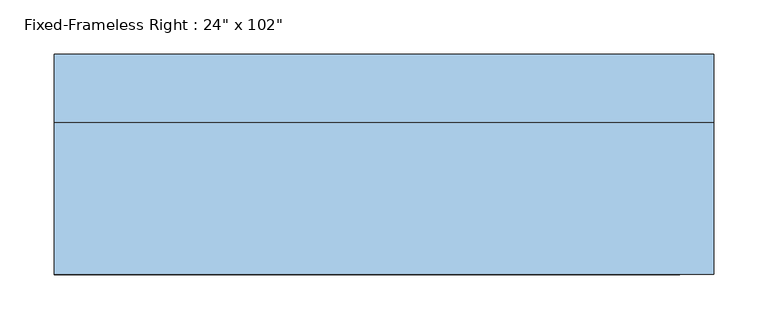
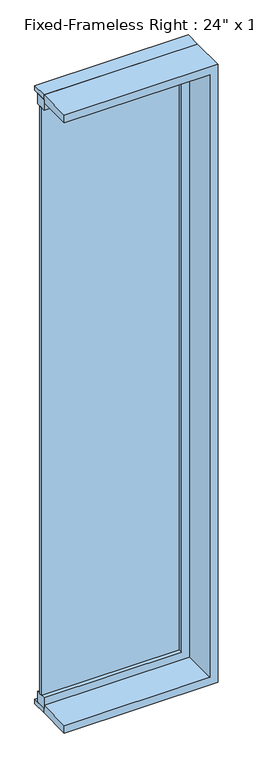
"""IFC4 building model written with IfcOpenShell, lengths in millimetres: window geometry."""

import ifcopenshell
import ifcopenshell.guid

model = None  # the IFC model being written
_history = None  # IfcOwnerHistory: only IFC2X3 demands one
_inside = {}  # id of a spatial element -> (the spatial element, [elements in it])
_under = {}  # id of a project, library or spatial element -> (it, [spatial elements below it])
_declared = {}  # id of a project -> (the project, [libraries it declares])
_typed = {}  # id of a type object -> (the type object, [elements of that type])
_made_of = {}  # id of a material, layer set ... -> (it, [elements and type objects made of it])


def new_model(schema):
    """Start an empty IFC model of exactly this schema.

    Asked for "IFC4X3", IfcOpenShell would pick the latest addendum, in which some entities
    have other attributes; the version numbers below select the first issue.
    IFC2X3 requires an IfcOwnerHistory on every rooted entity: one is made here for all.
    """
    global model, _history
    if schema == "IFC4X3":
        model = ifcopenshell.file(schema_version=(4, 3, 0, 0))
    else:
        model = ifcopenshell.file(schema=schema)
    _inside.clear()
    _under.clear()
    _declared.clear()
    _typed.clear()
    _made_of.clear()
    _history = None
    if model.schema == "IFC2X3":
        org = make("IfcOrganization", Name="unknown")
        user = make(
            "IfcPersonAndOrganization",
            ThePerson=make("IfcPerson", FamilyName="unknown"),
            TheOrganization=org,
        )
        app = make(
            "IfcApplication",
            ApplicationDeveloper=org,
            Version="unknown",
            ApplicationFullName="unknown",
            ApplicationIdentifier="unknown",
        )
        _history = make(
            "IfcOwnerHistory",
            OwningUser=user,
            OwningApplication=app,
            ChangeAction="ADDED",
            CreationDate=0,
        )
    return model


def make(cls, **values):
    """One entity of the class cls with the attributes given. An attribute that is None is left unset."""
    return model.create_entity(
        cls, **{name: value for name, value in values.items() if value is not None}
    )


def rooted(cls, **values):
    """An entity with a GlobalId (a new one), such as an element, a storey or a relation."""
    return make(cls, GlobalId=ifcopenshell.guid.new(), OwnerHistory=_history, **values)


def si_unit(unit_type, name, prefix=None):
    """IfcSIUnit, for example si_unit("LENGTHUNIT", "METRE", prefix="MILLI")."""
    return make("IfcSIUnit", UnitType=unit_type, Prefix=prefix, Name=name)


def assignment(units):
    """IfcUnitAssignment: the units of a project."""
    return None if units is None else make("IfcUnitAssignment", Units=units)


def point(xyz):
    """IfcCartesianPoint."""
    return None if xyz is None else make("IfcCartesianPoint", Coordinates=xyz)


def direction(xyz):
    """IfcDirection."""
    return None if xyz is None else make("IfcDirection", DirectionRatios=xyz)


def frame(location, z_axis=None, x_axis=None):
    """IfcAxis2Placement3D, a coordinate frame: its origin and axes. An axis left out is left unset."""
    return make(
        "IfcAxis2Placement3D",
        Location=point(location),
        Axis=direction(z_axis),
        RefDirection=direction(x_axis),
    )


def origin():
    """The frame at (0, 0, 0) with its axes left unset."""
    return frame((0.0, 0.0, 0.0))


def place(relative_to, where):
    """IfcLocalPlacement: puts the frame where relative to a parent placement (None: the world)."""
    return make(
        "IfcLocalPlacement", PlacementRelTo=relative_to, RelativePlacement=where
    )


def context(
    kind, dimensions, precision=None, world=None, true_north=None, identifier=None
):
    """IfcGeometricRepresentationContext, for example the 3D "Model" context."""
    return make(
        "IfcGeometricRepresentationContext",
        ContextIdentifier=identifier,
        ContextType=kind,
        CoordinateSpaceDimension=dimensions,
        Precision=precision,
        WorldCoordinateSystem=world,
        TrueNorth=true_north,
    )


def project(units=None, contexts=None):
    """IfcProject with its units and contexts."""
    return rooted(
        "IfcProject",
        Name="project",
        RepresentationContexts=contexts,
        UnitsInContext=assignment(units),
    )


def spatial(cls, under=None, at=None, **own):
    """A site, building, storey or space (cls), placed at a placement, below another one or the project."""
    s = rooted(cls, ObjectPlacement=at, **own)
    if under is not None:
        _under.setdefault(under.id(), (under, []))[1].append(s)
    return s


def polyline(points):
    """IfcPolyline through the points."""
    return make("IfcPolyline", Points=[point(p) for p in points])


def outline(outer, holes=None, kind="AREA"):
    """IfcArbitraryClosedProfileDef: a profile drawn as a closed curve; with holes, ...WithVoids."""
    if holes is None:
        return make("IfcArbitraryClosedProfileDef", ProfileType=kind, OuterCurve=outer)
    return make(
        "IfcArbitraryProfileDefWithVoids",
        ProfileType=kind,
        OuterCurve=outer,
        InnerCurves=holes,
    )


def extrude(swept, where, along, depth):
    """IfcExtrudedAreaSolid: the profile swept, set in the frame where, extruded along a direction by depth."""
    return make(
        "IfcExtrudedAreaSolid",
        SweptArea=swept,
        Position=where,
        ExtrudedDirection=direction(along),
        Depth=depth,
    )


def shape(context_of_items, identifier, shape_type, items):
    """IfcShapeRepresentation: the items that make up one representation, for example the "Body"."""
    return make(
        "IfcShapeRepresentation",
        ContextOfItems=context_of_items,
        RepresentationIdentifier=identifier,
        RepresentationType=shape_type,
        Items=items,
    )


def source(mapping_origin, context_of_items, identifier, shape_type, items):
    """IfcRepresentationMap: a shape defined once, which mapped items show again and again."""
    return make(
        "IfcRepresentationMap",
        MappingOrigin=mapping_origin,
        MappedRepresentation=shape(context_of_items, identifier, shape_type, items),
    )


def transform(
    local_origin,
    x_axis=None,
    y_axis=None,
    z_axis=None,
    scale=None,
    scale2=None,
    scale3=None,
    uniform=True,
):
    """IfcCartesianTransformationOperator3D, or its non-uniform kind. x_axis, y_axis, z_axis: its Axis1, 2, 3."""
    if uniform:
        return make(
            "IfcCartesianTransformationOperator3D",
            Axis1=direction(x_axis),
            Axis2=direction(y_axis),
            LocalOrigin=point(local_origin),
            Scale=scale,
            Axis3=direction(z_axis),
        )
    return make(
        "IfcCartesianTransformationOperator3DnonUniform",
        Axis1=direction(x_axis),
        Axis2=direction(y_axis),
        LocalOrigin=point(local_origin),
        Scale=scale,
        Axis3=direction(z_axis),
        Scale2=scale2,
        Scale3=scale3,
    )


def mapped(mapping_source, mapping_target):
    """IfcMappedItem: shows the shape of a source again, moved by a transform."""
    return make(
        "IfcMappedItem", MappingSource=mapping_source, MappingTarget=mapping_target
    )


def made_of(thing, what):
    """Note that an element or type object is made of a material, layer set ...; save() writes the relation."""
    if what is not None:
        _made_of.setdefault(what.id(), (what, []))[1].append(thing)
    return thing


def element(
    cls,
    number,
    at=None,
    inside=None,
    cuts=None,
    type_object=None,
    material=None,
    context=None,
    identifier="Body",
    shape_type=None,
    held_by="IfcProductDefinitionShape",
    body=None,
    shapes=None,
    **own,
):
    """One element of the class cls, such as IfcWall. Its Tag is "e" and its number.

    at: its placement. inside: the storey or other place that contains it. cuts: it is an
    opening in that element (IfcRelVoidsElement). A single representation is given by context,
    identifier, shape_type and body (its items); several are given by shapes. held_by: the class
    of the entity that holds the representations. save() writes the other relations.
    """
    e = rooted(cls, Tag="e%d" % number, ObjectPlacement=at, **own)
    if body is not None:
        shapes = [shape(context, identifier, shape_type, body)]
    if shapes is not None:
        e.Representation = make(held_by, Representations=shapes)
    if inside is not None:
        _inside.setdefault(inside.id(), (inside, []))[1].append(e)
    if cuts is not None:
        rooted(
            "IfcRelVoidsElement", RelatingBuildingElement=cuts, RelatedOpeningElement=e
        )
    if type_object is not None:
        _typed.setdefault(type_object.id(), (type_object, []))[1].append(e)
    return made_of(e, material)


def aggregate(whole, parts):
    """IfcRelAggregates: a whole, such as a stair, and the parts it consists of."""
    return rooted("IfcRelAggregates", RelatingObject=whole, RelatedObjects=parts)


def save(model, path):
    """Write the relations noted so far, then the file.

    IfcRelAggregates (storeys below a building ...), IfcRelContainedInSpatialStructure (elements
    in a storey), IfcRelDefinesByType, IfcRelAssociatesMaterial and IfcRelDeclares: one each for
    every whole, place, type object, material and project.
    """
    for whole, parts in _under.values():
        aggregate(whole, parts)
    for where, things in _inside.values():
        rooted(
            "IfcRelContainedInSpatialStructure",
            RelatedElements=things,
            RelatingStructure=where,
        )
    for kind, things in _typed.values():
        rooted("IfcRelDefinesByType", RelatedObjects=things, RelatingType=kind)
    for what, things in _made_of.values():
        rooted("IfcRelAssociatesMaterial", RelatedObjects=things, RelatingMaterial=what)
    for by, libraries in _declared.values():
        rooted("IfcRelDeclares", RelatingContext=by, RelatedDefinitions=libraries)
    model.write(path)


def window_ec3e7d3e(model_context):
    return source(origin(), model_context, "Body", "SweptSolid", [
        extrude(outline(polyline([(203.2, 53.975), (-342.9, 53.975), (-342.9, 66.675), (203.2, 66.675), (203.2, 53.975)])), frame((0.0, 0.0, 368.3), z_axis=(0.0, 0.0, 1.0), x_axis=(1.0, 0.0, 0.0)), (0.0, 0.0, 1.0), 2463.8),
        extrude(outline(polyline([(2876.55, -342.9), (2832.1, -342.9), (2832.1, 203.2), (368.3, 203.2), (368.3, -342.9), (323.85, -342.9), (323.85, 247.65), (2876.55, 247.65), (2876.55, -342.9)])), frame((0.0, 38.1, 0.0), z_axis=(0.0, 1.0, 0.0), x_axis=(0.0, 0.0, 1.0)), (0.0, 0.0, 1.0), 44.45),
        extrude(outline(polyline([(2895.6, -342.9), (2863.85, -342.9), (2863.85, 234.95), (336.55, 234.95), (336.55, -342.9), (304.8, -342.9), (304.8, 266.7), (2895.6, 266.7), (2895.6, -342.9)])), frame((0.0, -101.6, 0.0), z_axis=(0.0, 1.0, 0.0), x_axis=(0.0, 0.0, 1.0)), (0.0, 0.0, 1.0), 139.7),
        extrude(outline(polyline([(2895.6, 266.7), (2895.6, -342.9), (2876.55, -342.9), (2876.55, 247.65), (323.85, 247.65), (323.85, -342.9), (304.8, -342.9), (304.8, 266.7), (2895.6, 266.7)])), frame((0.0, 38.1, 0.0), z_axis=(0.0, 1.0, 0.0), x_axis=(0.0, 0.0, 1.0)), (0.0, 0.0, 1.0), 63.5),
    ])


if __name__ == "__main__":
    model = new_model("IFC4")
    model_context = context("Model", 3, world=origin())
    ifc_project = project(units=[si_unit("LENGTHUNIT", "METRE", prefix="MILLI")], contexts=[model_context])
    site = spatial("IfcSite", under=ifc_project)
    building = spatial("IfcBuilding", under=site)
    placement = place(None, origin())
    window_shape = window_ec3e7d3e(model_context)
    element("IfcWindow", 1, ObjectType="Fixed-Frameless Right : 24\" x 102\"", at=placement, inside=building, context=model_context, shape_type="MappedRepresentation", body=[
        mapped(window_shape, transform((0.0, 0.0, 0.0), x_axis=(1.0, 0.0, 0.0), y_axis=(0.0, 1.0, 0.0), z_axis=(0.0, 0.0, 1.0))),
    ])
    save(model, "model.ifc")

# Revit data of these elements
# Type "Fixed-Frameless Right : 24\" x 102\""
#   Type Mark = "59"
#   Assembly Code = "B2020100"
#   Height = 8' - 6"
#   Default Sill Height = 1' - 0"
#   Width = 2' - 0"
#   Window Inset = 0' - 0 3/4"
#   Glass Pane Material = Glass
#   Sash Material = Sash
#   Wall Closure = (empty or 0)
# Element 1 (IfcWindow, "Fixed-Frameless Right : 24\" x 102\"")
#   Materials on its faces: "Sash", "Glass"
# Materials
#   "Glass": class "Glass", colour RGB 0 128 192, transparency 0.75
#   "Sash": class "Wood", colour RGB 224 178 126, transparency 0
